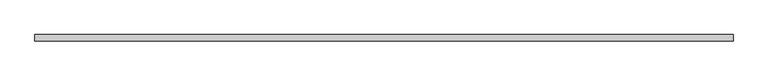
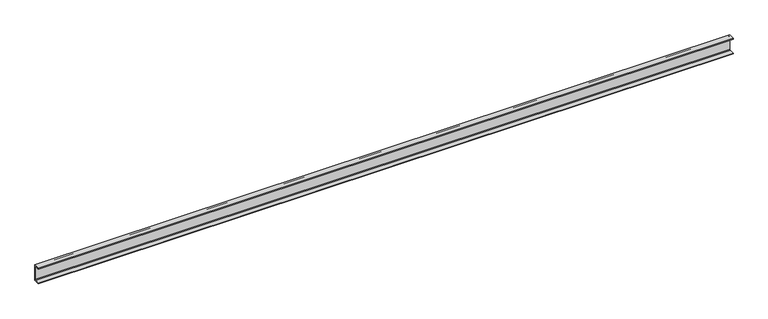
"""IFC4 building model written with IfcOpenShell, lengths in millimetres: beam geometry, С-образный профиль с параллельными полками (ГОСТ 8240-89) Балки : [ 20P."""

from ifc_helpers import new_model, si_unit, point, frame, frame_2d, origin, place, context, project, spatial, polyline, circle_curve, trimmed, segment, composite_curve, outline, extrude, source, transform, mapped, element, save


def beam_97961db2(model_context):
    return source(origin(), model_context, "Body", "SweptSolid", [
        extrude(outline(composite_curve([segment(polyline([(23.0, 100.0), (23.0, -100.0), (-53.0, -100.0), (-53.0, -91.0), (8.3, -91.0)]), True, "CONTINUOUS"), segment(trimmed(circle_curve(frame_2d((8.3, -81.5)), 9.5), [point((8.3, -91.0))], [point((17.8, -81.5))], True, "CARTESIAN"), True, "CONTINUOUS"), segment(polyline([(17.8, -81.5), (17.8, 81.5)]), True, "CONTINUOUS"), segment(trimmed(circle_curve(frame_2d((8.3, 81.5)), 9.5), [point((17.8, 81.5))], [point((8.3, 91.0))], True, "CARTESIAN"), True, "CONTINUOUS"), segment(polyline([(8.3, 91.0), (-53.0, 91.0), (-53.0, 100.0), (23.0, 100.0)]), True, "CONTINUOUS")], self_intersect=False)), frame((-4250.0, 0.0, 0.0), z_axis=(1.0, 0.0, 0.0), x_axis=(0.0, 1.0, 0.0)), (0.0, 0.0, 1.0), 8500.0),
    ])


if __name__ == "__main__":
    model = new_model("IFC4")
    model_context = context("Model", 3, world=origin())
    ifc_project = project(units=[si_unit("LENGTHUNIT", "METRE", prefix="MILLI")], contexts=[model_context])
    site = spatial("IfcSite", under=ifc_project)
    building = spatial("IfcBuilding", under=site)
    placement = place(None, origin())
    beam_shape = beam_97961db2(model_context)
    element("IfcBeam", 1, ObjectType="С-образный профиль с параллельными полками (ГОСТ 8240-89) Балки : [ 20P", at=placement, inside=building, context=model_context, shape_type="MappedRepresentation", body=[
        mapped(beam_shape, transform((0.0, 0.0, 0.0), x_axis=(1.0, 0.0, 0.0), y_axis=(0.0, 1.0, 0.0), z_axis=(0.0, 0.0, 1.0))),
    ])
    save(model, "model.ifc")

# Revit data of these elements
# Type "С-образный профиль с параллельными полками (ГОСТ 8240-89) Балки : [ 20P"
#   tf = 9 mm
#   ra = 9.5 mm
#   W = 0.180442
#   Vz = 100 mm
#   Vy = 53 mm
#   Vpz = 100 mm
#   Vpy = 23 mm
#   Length [instance default] = 1500 mm
#   bf = 76 mm
#   d = 200 mm
#   tw = 5.2 mm
#   A = 0.00234 m²
#   Structural Material [instance default] = Металл - Сталь - 345 МПa
#   Assembly Code = ""
# Element 1 (IfcBeam, "С-образный профиль с параллельными полками (ГОСТ 8240-89) Балки : [ 20P")
#   Structural Material = C245
#   Materials on its faces: "C245"
# Materials
#   "Металл - Сталь - 345 МПa": class "Металл", colour RGB 247 247 247, transparency 0
#   "C245": class "Не назначено", colour RGB 0 0 0, transparency 0
